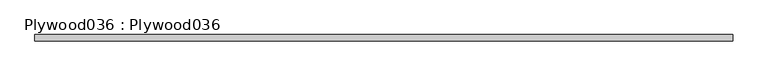
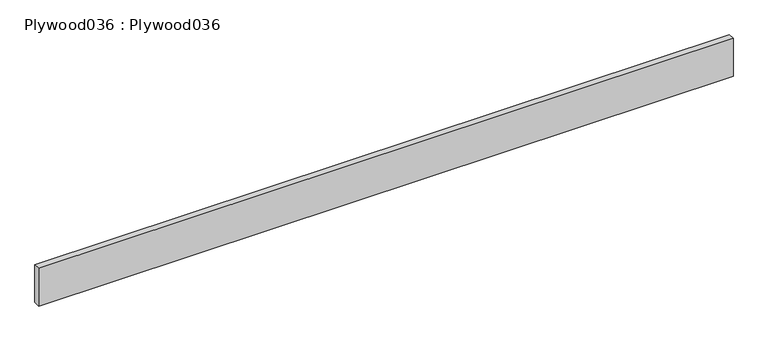
"""IFC4 building model written with IfcOpenShell, lengths in millimetres: proxy geometry, Plywood036 : Plywood036."""

from ifc_helpers import new_model, si_unit, frame, origin, place, context, project, spatial, polyline, outline, extrude, source, transform, mapped, element, save


def plywood036_plywood036_3faf7db6(model_context):
    return source(origin(), model_context, "Body", "SweptSolid", [
        extrude(outline(polyline([(14383.0178845, -5345.4165039), (14383.0178845, -5363.3725586), (12383.0178845, -5363.3725586), (12383.0178845, -5345.4165039), (14383.0178845, -5345.4165039)])), frame((0.0, 0.0, 42661.0807603), z_axis=(0.0, 0.0, 1.0), x_axis=(1.0, 0.0, 0.0)), (0.0, 0.0, 1.0), 114.3),
    ])


if __name__ == "__main__":
    model = new_model("IFC4")
    model_context = context("Model", 3, world=origin())
    ifc_project = project(units=[si_unit("LENGTHUNIT", "METRE", prefix="MILLI")], contexts=[model_context])
    site = spatial("IfcSite", under=ifc_project)
    building = spatial("IfcBuilding", under=site)
    placement = place(None, origin())
    plywood036_plywood036_shape = plywood036_plywood036_3faf7db6(model_context)
    element("IfcBuildingElementProxy", 1, Name="Plywood036 : Plywood036", ObjectType="Plywood036 : Plywood036", at=placement, inside=building, context=model_context, shape_type="MappedRepresentation", body=[
        mapped(plywood036_plywood036_shape, transform((0.0, 0.0, 0.0), x_axis=(1.0, 0.0, 0.0), y_axis=(0.0, 1.0, 0.0), z_axis=(0.0, 0.0, 1.0))),
    ])
    save(model, "model.ifc")

# Revit data of these elements
# Type "Plywood036 : Plywood036"
#   NameOverride = "Plywood036"
# Element 1 (IfcBuildingElementProxy, "Plywood036 : Plywood036")
#   Materials on its faces: "CDX PLYWOOD - SEE STRUCTURAL DWGS"
# Materials
#   "CDX PLYWOOD - SEE STRUCTURAL DWGS": class "Unassigned", colour RGB 177 130 114, transparency 0, Cost = 0
